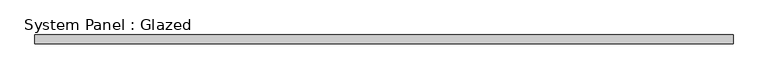
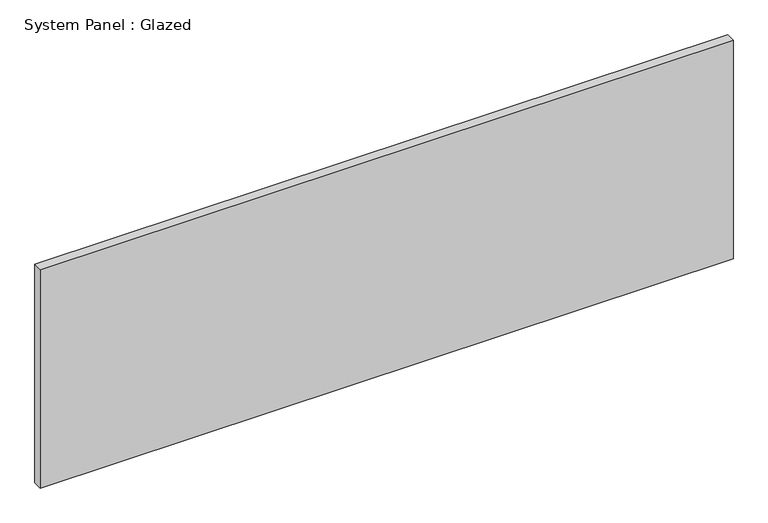
"""IFC4 building model written with IfcOpenShell, lengths in millimetres: plate geometry, System Panel : Glazed."""

from ifc_helpers import new_model, si_unit, origin, origin_with_axes, place, context, project, spatial, polyline, outline, extrude, source, transform, mapped, element, save


def system_panel_glazed_280cb7dc(model_context):
    return source(origin(), model_context, "Body", "SweptSolid", [
        extrude(outline(polyline([(975.0, 24.5), (-975.0, 24.5), (-975.0, 49.5), (975.0, 49.5), (975.0, 24.5)])), origin_with_axes(), (0.0, 0.0, 1.0), 650.0),
    ])


if __name__ == "__main__":
    model = new_model("IFC4")
    model_context = context("Model", 3, world=origin())
    ifc_project = project(units=[si_unit("LENGTHUNIT", "METRE", prefix="MILLI")], contexts=[model_context])
    site = spatial("IfcSite", under=ifc_project)
    building = spatial("IfcBuilding", under=site)
    placement = place(None, origin())
    system_panel_glazed_shape = system_panel_glazed_280cb7dc(model_context)
    element("IfcPlate", 1, ObjectType="System Panel : Glazed", at=placement, inside=building, context=model_context, shape_type="MappedRepresentation", body=[
        mapped(system_panel_glazed_shape, transform((0.0, 0.0, 0.0), x_axis=(1.0, 0.0, 0.0), y_axis=(0.0, 1.0, 0.0), z_axis=(0.0, 0.0, 1.0))),
    ])
    save(model, "model.ifc")

# Revit data of these elements
# Element 1 (IfcPlate, "System Panel : Glazed")
#   Materials on its faces: "Glass"
# Materials
#   "Glass": class "Glass", colour RGB 0 128 192, transparency 0.9
